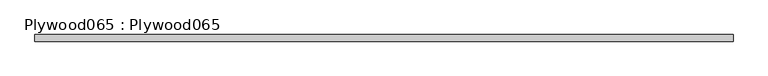
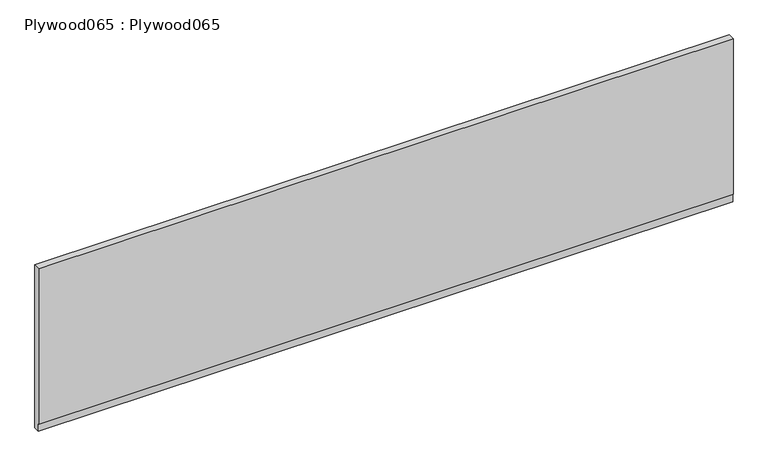
"""IFC4 building model written with IfcOpenShell, lengths in millimetres: proxy geometry, Plywood065 : Plywood065."""

from ifc_helpers import new_model, si_unit, frame, origin, place, context, project, spatial, polyline, outline, extrude, source, transform, mapped, element, save


def plywood065_plywood065_2c9fae8a(model_context):
    return source(origin(), model_context, "Body", "SweptSolid", [
        extrude(outline(polyline([(-5543.3480267, 40210.7296087), (-5543.3480267, 39714.0839618), (-5561.1180267, 39714.0839618), (-5561.1180267, 39736.6047233), (-5562.3980267, 39736.6047233), (-5562.3980267, 40210.7296087), (-5543.3480267, 40210.7296087)])), frame((12382.7678845, 0.0, 0.0), z_axis=(1.0, 0.0, 0.0), x_axis=(0.0, 1.0, 0.0)), (0.0, 0.0, 1.0), 2000.25),
    ])


if __name__ == "__main__":
    model = new_model("IFC4")
    model_context = context("Model", 3, world=origin())
    ifc_project = project(units=[si_unit("LENGTHUNIT", "METRE", prefix="MILLI")], contexts=[model_context])
    site = spatial("IfcSite", under=ifc_project)
    building = spatial("IfcBuilding", under=site)
    placement = place(None, origin())
    plywood065_plywood065_shape = plywood065_plywood065_2c9fae8a(model_context)
    element("IfcBuildingElementProxy", 1, Name="Plywood065 : Plywood065", ObjectType="Plywood065 : Plywood065", at=placement, inside=building, context=model_context, shape_type="MappedRepresentation", body=[
        mapped(plywood065_plywood065_shape, transform((0.0, 0.0, 0.0), x_axis=(1.0, 0.0, 0.0), y_axis=(0.0, 1.0, 0.0), z_axis=(0.0, 0.0, 1.0))),
    ])
    save(model, "model.ifc")

# Revit data of these elements
# Type "Plywood065 : Plywood065"
#   NameOverride = "Plywood065"
# Element 1 (IfcBuildingElementProxy, "Plywood065 : Plywood065")
#   Materials on its faces: "7/8\" SMOOTH TROWEL EXTERIOR STUCCO"
# Materials
#   "7/8\" SMOOTH TROWEL EXTERIOR STUCCO": class "Unassigned", colour RGB 255 255 255, transparency 0, Cost = 0
